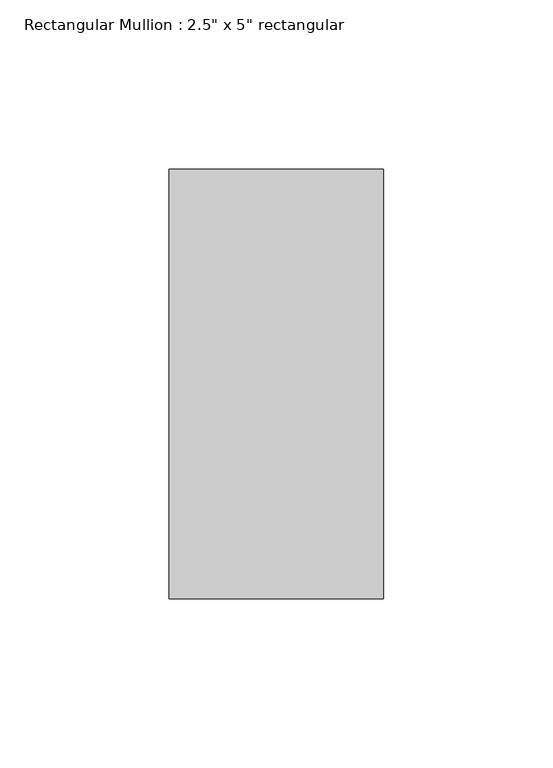
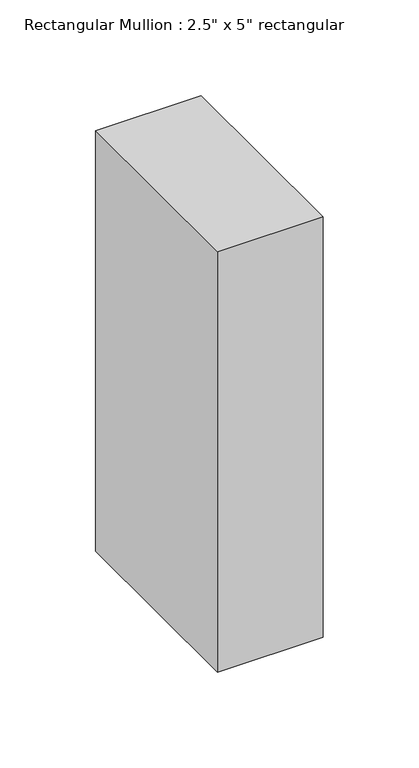
"""IFC4 building model written with IfcOpenShell, lengths in millimetres: member geometry."""

from ifc_helpers import new_model, si_unit, frame, origin, place, context, project, spatial, polyline, outline, extrude, source, transform, mapped, element, save


def member_f5b3432e(model_context):
    return source(origin(), model_context, "Body", "SweptSolid", [
        extrude(outline(polyline([(0.0, 63.5), (0.0, -63.5), (-63.5, -63.5), (-63.5, 63.5), (0.0, 63.5)])), frame((0.0, 0.0, -267.49375), z_axis=(0.0, 0.0, 1.0), x_axis=(1.0, 0.0, 0.0)), (0.0, 0.0, 1.0), 267.49375),
    ])


if __name__ == "__main__":
    model = new_model("IFC4")
    model_context = context("Model", 3, world=origin())
    ifc_project = project(units=[si_unit("LENGTHUNIT", "METRE", prefix="MILLI")], contexts=[model_context])
    site = spatial("IfcSite", under=ifc_project)
    building = spatial("IfcBuilding", under=site)
    placement = place(None, origin())
    member_shape = member_f5b3432e(model_context)
    element("IfcMember", 1, ObjectType="Rectangular Mullion : 2.5\" x 5\" rectangular", at=placement, inside=building, context=model_context, shape_type="MappedRepresentation", body=[
        mapped(member_shape, transform((0.0, 0.0, 0.0), x_axis=(1.0, 0.0, 0.0), y_axis=(0.0, 1.0, 0.0), z_axis=(0.0, 0.0, 1.0))),
    ])
    save(model, "model.ifc")

# Revit data of these elements
# Type "Rectangular Mullion : 2.5\" x 5\" rectangular"
#   built-in parameter 1007304 = 0.416667 (stored number, unit not read)
#   built-in parameter 1007301 = 0.104167 (stored number, unit not read)
#   built-in parameter 1007300 = 0.104167 (stored number, unit not read)
# Element 1 (IfcMember, "Rectangular Mullion : 2.5\" x 5\" rectangular")
#   Materials on its faces: "Metal - Aluminum"
# Materials
#   "Metal - Aluminum": class "Metal", colour RGB 140 140 140, transparency 0
